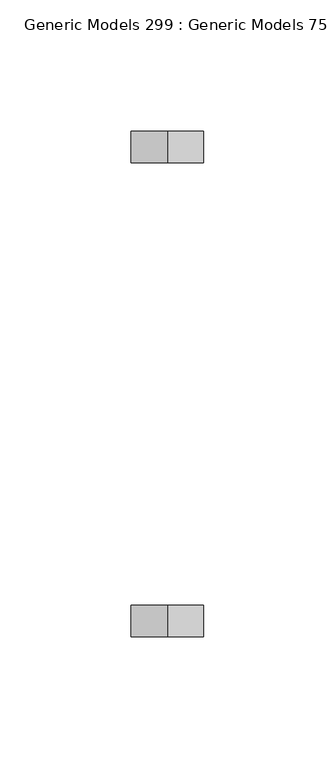
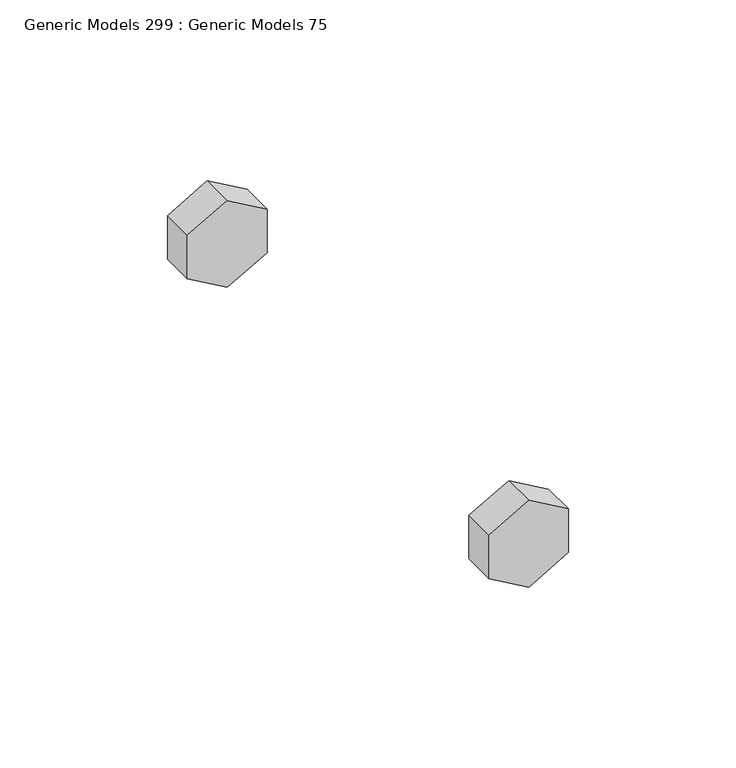
"""IFC4 building model written with IfcOpenShell, lengths in millimetres: proxy geometry, Generic Models 299 : Generic Models 75."""

import ifcopenshell
import ifcopenshell.guid

model = None  # the IFC model being written
_history = None  # IfcOwnerHistory: only IFC2X3 demands one
_inside = {}  # id of a spatial element -> (the spatial element, [elements in it])
_under = {}  # id of a project, library or spatial element -> (it, [spatial elements below it])
_declared = {}  # id of a project -> (the project, [libraries it declares])
_typed = {}  # id of a type object -> (the type object, [elements of that type])
_made_of = {}  # id of a material, layer set ... -> (it, [elements and type objects made of it])


def new_model(schema):
    """Start an empty IFC model of exactly this schema.

    Asked for "IFC4X3", IfcOpenShell would pick the latest addendum, in which some entities
    have other attributes; the version numbers below select the first issue.
    IFC2X3 requires an IfcOwnerHistory on every rooted entity: one is made here for all.
    """
    global model, _history
    if schema == "IFC4X3":
        model = ifcopenshell.file(schema_version=(4, 3, 0, 0))
    else:
        model = ifcopenshell.file(schema=schema)
    _inside.clear()
    _under.clear()
    _declared.clear()
    _typed.clear()
    _made_of.clear()
    _history = None
    if model.schema == "IFC2X3":
        org = make("IfcOrganization", Name="unknown")
        user = make(
            "IfcPersonAndOrganization",
            ThePerson=make("IfcPerson", FamilyName="unknown"),
            TheOrganization=org,
        )
        app = make(
            "IfcApplication",
            ApplicationDeveloper=org,
            Version="unknown",
            ApplicationFullName="unknown",
            ApplicationIdentifier="unknown",
        )
        _history = make(
            "IfcOwnerHistory",
            OwningUser=user,
            OwningApplication=app,
            ChangeAction="ADDED",
            CreationDate=0,
        )
    return model


def make(cls, **values):
    """One entity of the class cls with the attributes given. An attribute that is None is left unset."""
    return model.create_entity(
        cls, **{name: value for name, value in values.items() if value is not None}
    )


def rooted(cls, **values):
    """An entity with a GlobalId (a new one), such as an element, a storey or a relation."""
    return make(cls, GlobalId=ifcopenshell.guid.new(), OwnerHistory=_history, **values)


def si_unit(unit_type, name, prefix=None):
    """IfcSIUnit, for example si_unit("LENGTHUNIT", "METRE", prefix="MILLI")."""
    return make("IfcSIUnit", UnitType=unit_type, Prefix=prefix, Name=name)


def assignment(units):
    """IfcUnitAssignment: the units of a project."""
    return None if units is None else make("IfcUnitAssignment", Units=units)


def point(xyz):
    """IfcCartesianPoint."""
    return None if xyz is None else make("IfcCartesianPoint", Coordinates=xyz)


def direction(xyz):
    """IfcDirection."""
    return None if xyz is None else make("IfcDirection", DirectionRatios=xyz)


def frame(location, z_axis=None, x_axis=None):
    """IfcAxis2Placement3D, a coordinate frame: its origin and axes. An axis left out is left unset."""
    return make(
        "IfcAxis2Placement3D",
        Location=point(location),
        Axis=direction(z_axis),
        RefDirection=direction(x_axis),
    )


def origin():
    """The frame at (0, 0, 0) with its axes left unset."""
    return frame((0.0, 0.0, 0.0))


def place(relative_to, where):
    """IfcLocalPlacement: puts the frame where relative to a parent placement (None: the world)."""
    return make(
        "IfcLocalPlacement", PlacementRelTo=relative_to, RelativePlacement=where
    )


def context(
    kind, dimensions, precision=None, world=None, true_north=None, identifier=None
):
    """IfcGeometricRepresentationContext, for example the 3D "Model" context."""
    return make(
        "IfcGeometricRepresentationContext",
        ContextIdentifier=identifier,
        ContextType=kind,
        CoordinateSpaceDimension=dimensions,
        Precision=precision,
        WorldCoordinateSystem=world,
        TrueNorth=true_north,
    )


def project(units=None, contexts=None):
    """IfcProject with its units and contexts."""
    return rooted(
        "IfcProject",
        Name="project",
        RepresentationContexts=contexts,
        UnitsInContext=assignment(units),
    )


def spatial(cls, under=None, at=None, **own):
    """A site, building, storey or space (cls), placed at a placement, below another one or the project."""
    s = rooted(cls, ObjectPlacement=at, **own)
    if under is not None:
        _under.setdefault(under.id(), (under, []))[1].append(s)
    return s


def polyline(points):
    """IfcPolyline through the points."""
    return make("IfcPolyline", Points=[point(p) for p in points])


def outline(outer, holes=None, kind="AREA"):
    """IfcArbitraryClosedProfileDef: a profile drawn as a closed curve; with holes, ...WithVoids."""
    if holes is None:
        return make("IfcArbitraryClosedProfileDef", ProfileType=kind, OuterCurve=outer)
    return make(
        "IfcArbitraryProfileDefWithVoids",
        ProfileType=kind,
        OuterCurve=outer,
        InnerCurves=holes,
    )


def extrude(swept, where, along, depth):
    """IfcExtrudedAreaSolid: the profile swept, set in the frame where, extruded along a direction by depth."""
    return make(
        "IfcExtrudedAreaSolid",
        SweptArea=swept,
        Position=where,
        ExtrudedDirection=direction(along),
        Depth=depth,
    )


def shape(context_of_items, identifier, shape_type, items):
    """IfcShapeRepresentation: the items that make up one representation, for example the "Body"."""
    return make(
        "IfcShapeRepresentation",
        ContextOfItems=context_of_items,
        RepresentationIdentifier=identifier,
        RepresentationType=shape_type,
        Items=items,
    )


def source(mapping_origin, context_of_items, identifier, shape_type, items):
    """IfcRepresentationMap: a shape defined once, which mapped items show again and again."""
    return make(
        "IfcRepresentationMap",
        MappingOrigin=mapping_origin,
        MappedRepresentation=shape(context_of_items, identifier, shape_type, items),
    )


def transform(
    local_origin,
    x_axis=None,
    y_axis=None,
    z_axis=None,
    scale=None,
    scale2=None,
    scale3=None,
    uniform=True,
):
    """IfcCartesianTransformationOperator3D, or its non-uniform kind. x_axis, y_axis, z_axis: its Axis1, 2, 3."""
    if uniform:
        return make(
            "IfcCartesianTransformationOperator3D",
            Axis1=direction(x_axis),
            Axis2=direction(y_axis),
            LocalOrigin=point(local_origin),
            Scale=scale,
            Axis3=direction(z_axis),
        )
    return make(
        "IfcCartesianTransformationOperator3DnonUniform",
        Axis1=direction(x_axis),
        Axis2=direction(y_axis),
        LocalOrigin=point(local_origin),
        Scale=scale,
        Axis3=direction(z_axis),
        Scale2=scale2,
        Scale3=scale3,
    )


def mapped(mapping_source, mapping_target):
    """IfcMappedItem: shows the shape of a source again, moved by a transform."""
    return make(
        "IfcMappedItem", MappingSource=mapping_source, MappingTarget=mapping_target
    )


def made_of(thing, what):
    """Note that an element or type object is made of a material, layer set ...; save() writes the relation."""
    if what is not None:
        _made_of.setdefault(what.id(), (what, []))[1].append(thing)
    return thing


def element(
    cls,
    number,
    at=None,
    inside=None,
    cuts=None,
    type_object=None,
    material=None,
    context=None,
    identifier="Body",
    shape_type=None,
    held_by="IfcProductDefinitionShape",
    body=None,
    shapes=None,
    **own,
):
    """One element of the class cls, such as IfcWall. Its Tag is "e" and its number.

    at: its placement. inside: the storey or other place that contains it. cuts: it is an
    opening in that element (IfcRelVoidsElement). A single representation is given by context,
    identifier, shape_type and body (its items); several are given by shapes. held_by: the class
    of the entity that holds the representations. save() writes the other relations.
    """
    e = rooted(cls, Tag="e%d" % number, ObjectPlacement=at, **own)
    if body is not None:
        shapes = [shape(context, identifier, shape_type, body)]
    if shapes is not None:
        e.Representation = make(held_by, Representations=shapes)
    if inside is not None:
        _inside.setdefault(inside.id(), (inside, []))[1].append(e)
    if cuts is not None:
        rooted(
            "IfcRelVoidsElement", RelatingBuildingElement=cuts, RelatedOpeningElement=e
        )
    if type_object is not None:
        _typed.setdefault(type_object.id(), (type_object, []))[1].append(e)
    return made_of(e, material)


def aggregate(whole, parts):
    """IfcRelAggregates: a whole, such as a stair, and the parts it consists of."""
    return rooted("IfcRelAggregates", RelatingObject=whole, RelatedObjects=parts)


def save(model, path):
    """Write the relations noted so far, then the file.

    IfcRelAggregates (storeys below a building ...), IfcRelContainedInSpatialStructure (elements
    in a storey), IfcRelDefinesByType, IfcRelAssociatesMaterial and IfcRelDeclares: one each for
    every whole, place, type object, material and project.
    """
    for whole, parts in _under.values():
        aggregate(whole, parts)
    for where, things in _inside.values():
        rooted(
            "IfcRelContainedInSpatialStructure",
            RelatedElements=things,
            RelatingStructure=where,
        )
    for kind, things in _typed.values():
        rooted("IfcRelDefinesByType", RelatedObjects=things, RelatingType=kind)
    for what, things in _made_of.values():
        rooted("IfcRelAssociatesMaterial", RelatedObjects=things, RelatingMaterial=what)
    for by, libraries in _declared.values():
        rooted("IfcRelDeclares", RelatingContext=by, RelatedDefinitions=libraries)
    model.write(path)


def generic_models_299_generic_models_75_51a980cc(model_context):
    return source(origin(), model_context, "Body", "SweptSolid", [
        extrude(outline(polyline([(269146.3182867, 31975.9942029), (269130.4817133, 31975.9942029), (269122.5634265, 31989.7090778), (269130.4817133, 32003.4239528), (269146.3182867, 32003.4239528), (269154.2365735, 31989.7090778), (269146.3182867, 31975.9942029)])), frame((0.0, 35373.9582942, 0.0), z_axis=(0.0, 1.0, 0.0), x_axis=(0.0, 0.0, 1.0)), (0.0, 0.0, 1.0), 11.90625),
        extrude(outline(polyline([(269146.3182867, 31975.9942029), (269130.4817133, 31975.9942029), (269122.5634265, 31989.7090778), (269130.4817133, 32003.4239528), (269146.3182867, 32003.4239528), (269154.2365735, 31989.7090778), (269146.3182867, 31975.9942029)])), frame((0.0, 35193.7770442, 0.0), z_axis=(0.0, 1.0, 0.0), x_axis=(0.0, 0.0, 1.0)), (0.0, 0.0, 1.0), 11.90625),
    ])


if __name__ == "__main__":
    model = new_model("IFC4")
    model_context = context("Model", 3, world=origin())
    ifc_project = project(units=[si_unit("LENGTHUNIT", "METRE", prefix="MILLI")], contexts=[model_context])
    site = spatial("IfcSite", under=ifc_project)
    building = spatial("IfcBuilding", under=site)
    placement = place(None, origin())
    generic_models_299_generic_models_75_shape = generic_models_299_generic_models_75_51a980cc(model_context)
    element("IfcBuildingElementProxy", 1, Name="Generic Models 299 : Generic Models 75", ObjectType="Generic Models 299 : Generic Models 75", at=placement, inside=building, context=model_context, shape_type="MappedRepresentation", body=[
        mapped(generic_models_299_generic_models_75_shape, transform((0.0, 0.0, 0.0), x_axis=(1.0, 0.0, 0.0), y_axis=(0.0, 1.0, 0.0), z_axis=(0.0, 0.0, 1.0))),
    ])
    save(model, "model.ifc")

# Revit data of these elements
# Element 1 (IfcBuildingElementProxy, "Generic Models 299 : Generic Models 75")
#   Materials on its faces: "3/4\" GALV. THRU BOLTS"
# Materials
#   "3/4\" GALV. THRU BOLTS": class "Generic", colour RGB 105 69 171, transparency 0, Cost = 0
